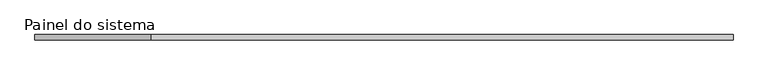
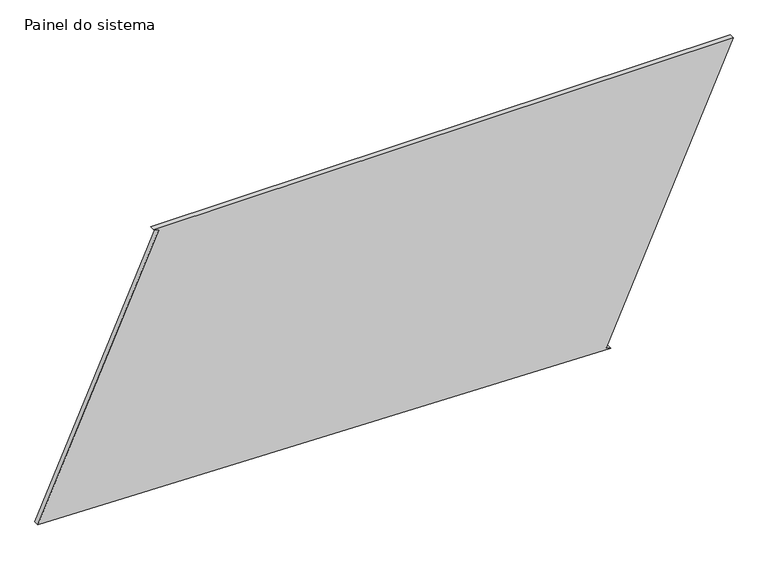
"""IFC4 building model written with IfcOpenShell, lengths in millimetres: plate geometry, Painel do sistema : Envidraçado."""

from ifc_helpers import new_model, si_unit, frame, origin, place, context, project, spatial, polyline, outline, extrude, source, transform, mapped, element, save


def painel_do_sistema_86205c73(model_context):
    return source(origin(), model_context, "Body", "SweptSolid", [
        extrude(outline(polyline([(0.0, 1086.4956147), (10.2299965, 1063.6844953), (1374.4117737, 1675.4727459), (1374.4117737, -1116.6183474), (1364.1817772, -1093.8072279), (67.1684736, -1675.4727459), (0.0, 1086.4956147)])), frame((0.0, 24.5, 0.0), z_axis=(0.0, 1.0, 0.0), x_axis=(0.0, 0.0, 1.0)), (0.0, 0.0, 1.0), 25.0),
    ])


if __name__ == "__main__":
    model = new_model("IFC4")
    model_context = context("Model", 3, world=origin())
    ifc_project = project(units=[si_unit("LENGTHUNIT", "METRE", prefix="MILLI")], contexts=[model_context])
    site = spatial("IfcSite", under=ifc_project)
    building = spatial("IfcBuilding", under=site)
    placement = place(None, origin())
    painel_do_sistema_shape = painel_do_sistema_86205c73(model_context)
    element("IfcPlate", 1, ObjectType="Painel do sistema : Envidraçado", at=placement, inside=building, context=model_context, shape_type="MappedRepresentation", body=[
        mapped(painel_do_sistema_shape, transform((0.0, 0.0, 0.0), x_axis=(1.0, 0.0, 0.0), y_axis=(0.0, 1.0, 0.0), z_axis=(0.0, 0.0, 1.0))),
    ])
    save(model, "model.ifc")

# Revit data of these elements
# Type "Painel do sistema : Envidraçado"
#   Construction Type Id = "GSP4R"
#   Analytic Construction = "Vidraça única Pilkington 1/8 pol"
#   Visual Light Transmittance = 0.9
#   Solar Heat Gain Coefficient = 0.86
#   Heat Transfer Coefficient (U) = 6.7069 W/(m²·K)
# Element 1 (IfcPlate, "Painel do sistema : Envidraçado")
#   Materials on its faces: "Vidro"
# Materials
#   "Vidro": class "Vidro", colour RGB 0 128 192, transparency 0.9, Description = "Vidro de sílica", Cost = 0
